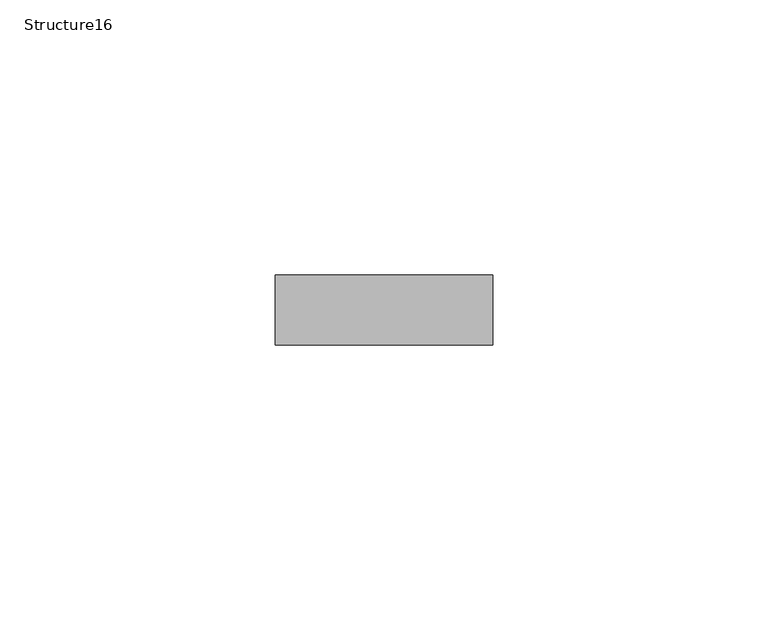
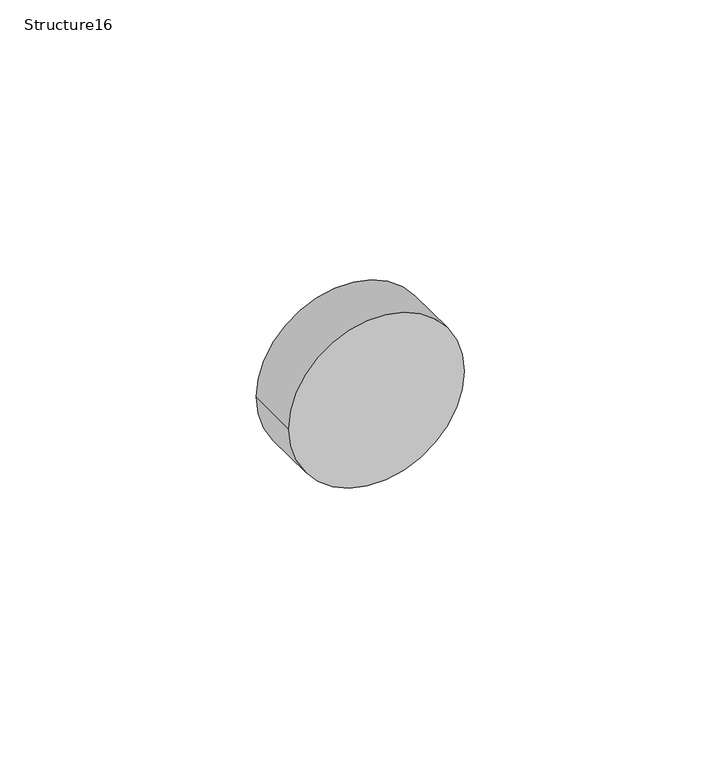
"""IFC4 building model written with IfcOpenShell, lengths in millimetres: proxy geometry, Structure16 : Structure668217137."""

from ifc_helpers import new_model, si_unit, point, frame, frame_2d, origin, place, context, project, spatial, circle_curve, trimmed, segment, composite_curve, outline, extrude, source, transform, mapped, element, save


def structure16_9385795e(model_context):
    return source(origin(), model_context, "Body", "SweptSolid", [
        extrude(outline(composite_curve([segment(trimmed(circle_curve(frame_2d((38047.8454063, 5185.7383658)), 19.7708678), [point((38047.8454063, 5165.967498))], [point((38047.8454063, 5205.5092336))], False, "CARTESIAN"), True, "CONTINUOUS"), segment(trimmed(circle_curve(frame_2d((38047.8454063, 5185.7383658)), 19.7708678), [point((38047.8454063, 5205.5092336))], [point((38047.8454063, 5165.967498))], False, "CARTESIAN"), True, "CONTINUOUS")], self_intersect=False)), frame((0.0, 1913.4572934, 0.0), z_axis=(0.0, 1.0, 0.0), x_axis=(0.0, 0.0, 1.0)), (0.0, 0.0, 1.0), 12.7),
    ])


if __name__ == "__main__":
    model = new_model("IFC4")
    model_context = context("Model", 3, world=origin())
    ifc_project = project(units=[si_unit("LENGTHUNIT", "METRE", prefix="MILLI")], contexts=[model_context])
    site = spatial("IfcSite", under=ifc_project)
    building = spatial("IfcBuilding", under=site)
    placement = place(None, origin())
    structure16_shape = structure16_9385795e(model_context)
    element("IfcBuildingElementProxy", 1, Name="Structure16 : Structure668217137", ObjectType="Structure16 : Structure668217137", at=placement, inside=building, context=model_context, shape_type="MappedRepresentation", body=[
        mapped(structure16_shape, transform((0.0, 0.0, 0.0), x_axis=(1.0, 0.0, 0.0), y_axis=(0.0, 1.0, 0.0), z_axis=(0.0, 0.0, 1.0))),
    ])
    save(model, "model.ifc")

# Revit data of these elements
# Type "Structure16 : Structure668217137"
#   NameOverride = "Structure668217137"
# Element 1 (IfcBuildingElementProxy, "Structure16 : Structure668217137")
#   Materials on its faces: "1.5\" DIA. STAINLESS STEEL RAILING"
# Materials
#   "1.5\" DIA. STAINLESS STEEL RAILING": class "Unassigned", colour RGB 128 128 128, transparency 0, Cost = 0
